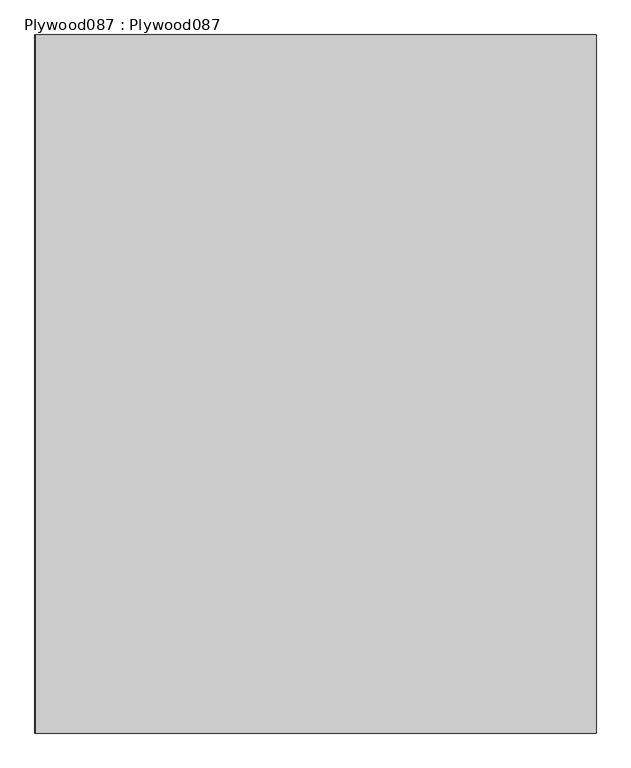
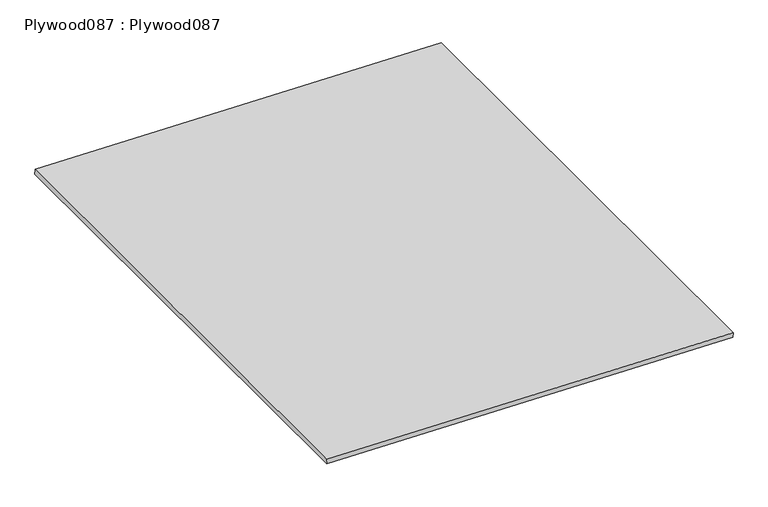
"""IFC4 building model written with IfcOpenShell, lengths in millimetres: proxy geometry, Plywood087 : Plywood087."""

import ifcopenshell
import ifcopenshell.guid

model = None  # the IFC model being written
_history = None  # IfcOwnerHistory: only IFC2X3 demands one
_inside = {}  # id of a spatial element -> (the spatial element, [elements in it])
_under = {}  # id of a project, library or spatial element -> (it, [spatial elements below it])
_declared = {}  # id of a project -> (the project, [libraries it declares])
_typed = {}  # id of a type object -> (the type object, [elements of that type])
_made_of = {}  # id of a material, layer set ... -> (it, [elements and type objects made of it])


def new_model(schema):
    """Start an empty IFC model of exactly this schema.

    Asked for "IFC4X3", IfcOpenShell would pick the latest addendum, in which some entities
    have other attributes; the version numbers below select the first issue.
    IFC2X3 requires an IfcOwnerHistory on every rooted entity: one is made here for all.
    """
    global model, _history
    if schema == "IFC4X3":
        model = ifcopenshell.file(schema_version=(4, 3, 0, 0))
    else:
        model = ifcopenshell.file(schema=schema)
    _inside.clear()
    _under.clear()
    _declared.clear()
    _typed.clear()
    _made_of.clear()
    _history = None
    if model.schema == "IFC2X3":
        org = make("IfcOrganization", Name="unknown")
        user = make(
            "IfcPersonAndOrganization",
            ThePerson=make("IfcPerson", FamilyName="unknown"),
            TheOrganization=org,
        )
        app = make(
            "IfcApplication",
            ApplicationDeveloper=org,
            Version="unknown",
            ApplicationFullName="unknown",
            ApplicationIdentifier="unknown",
        )
        _history = make(
            "IfcOwnerHistory",
            OwningUser=user,
            OwningApplication=app,
            ChangeAction="ADDED",
            CreationDate=0,
        )
    return model


def make(cls, **values):
    """One entity of the class cls with the attributes given. An attribute that is None is left unset."""
    return model.create_entity(
        cls, **{name: value for name, value in values.items() if value is not None}
    )


def rooted(cls, **values):
    """An entity with a GlobalId (a new one), such as an element, a storey or a relation."""
    return make(cls, GlobalId=ifcopenshell.guid.new(), OwnerHistory=_history, **values)


def si_unit(unit_type, name, prefix=None):
    """IfcSIUnit, for example si_unit("LENGTHUNIT", "METRE", prefix="MILLI")."""
    return make("IfcSIUnit", UnitType=unit_type, Prefix=prefix, Name=name)


def assignment(units):
    """IfcUnitAssignment: the units of a project."""
    return None if units is None else make("IfcUnitAssignment", Units=units)


def point(xyz):
    """IfcCartesianPoint."""
    return None if xyz is None else make("IfcCartesianPoint", Coordinates=xyz)


def direction(xyz):
    """IfcDirection."""
    return None if xyz is None else make("IfcDirection", DirectionRatios=xyz)


def frame(location, z_axis=None, x_axis=None):
    """IfcAxis2Placement3D, a coordinate frame: its origin and axes. An axis left out is left unset."""
    return make(
        "IfcAxis2Placement3D",
        Location=point(location),
        Axis=direction(z_axis),
        RefDirection=direction(x_axis),
    )


def origin():
    """The frame at (0, 0, 0) with its axes left unset."""
    return frame((0.0, 0.0, 0.0))


def place(relative_to, where):
    """IfcLocalPlacement: puts the frame where relative to a parent placement (None: the world)."""
    return make(
        "IfcLocalPlacement", PlacementRelTo=relative_to, RelativePlacement=where
    )


def context(
    kind, dimensions, precision=None, world=None, true_north=None, identifier=None
):
    """IfcGeometricRepresentationContext, for example the 3D "Model" context."""
    return make(
        "IfcGeometricRepresentationContext",
        ContextIdentifier=identifier,
        ContextType=kind,
        CoordinateSpaceDimension=dimensions,
        Precision=precision,
        WorldCoordinateSystem=world,
        TrueNorth=true_north,
    )


def project(units=None, contexts=None):
    """IfcProject with its units and contexts."""
    return rooted(
        "IfcProject",
        Name="project",
        RepresentationContexts=contexts,
        UnitsInContext=assignment(units),
    )


def spatial(cls, under=None, at=None, **own):
    """A site, building, storey or space (cls), placed at a placement, below another one or the project."""
    s = rooted(cls, ObjectPlacement=at, **own)
    if under is not None:
        _under.setdefault(under.id(), (under, []))[1].append(s)
    return s


def polyline(points):
    """IfcPolyline through the points."""
    return make("IfcPolyline", Points=[point(p) for p in points])


def outline(outer, holes=None, kind="AREA"):
    """IfcArbitraryClosedProfileDef: a profile drawn as a closed curve; with holes, ...WithVoids."""
    if holes is None:
        return make("IfcArbitraryClosedProfileDef", ProfileType=kind, OuterCurve=outer)
    return make(
        "IfcArbitraryProfileDefWithVoids",
        ProfileType=kind,
        OuterCurve=outer,
        InnerCurves=holes,
    )


def extrude(swept, where, along, depth):
    """IfcExtrudedAreaSolid: the profile swept, set in the frame where, extruded along a direction by depth."""
    return make(
        "IfcExtrudedAreaSolid",
        SweptArea=swept,
        Position=where,
        ExtrudedDirection=direction(along),
        Depth=depth,
    )


def shape(context_of_items, identifier, shape_type, items):
    """IfcShapeRepresentation: the items that make up one representation, for example the "Body"."""
    return make(
        "IfcShapeRepresentation",
        ContextOfItems=context_of_items,
        RepresentationIdentifier=identifier,
        RepresentationType=shape_type,
        Items=items,
    )


def source(mapping_origin, context_of_items, identifier, shape_type, items):
    """IfcRepresentationMap: a shape defined once, which mapped items show again and again."""
    return make(
        "IfcRepresentationMap",
        MappingOrigin=mapping_origin,
        MappedRepresentation=shape(context_of_items, identifier, shape_type, items),
    )


def transform(
    local_origin,
    x_axis=None,
    y_axis=None,
    z_axis=None,
    scale=None,
    scale2=None,
    scale3=None,
    uniform=True,
):
    """IfcCartesianTransformationOperator3D, or its non-uniform kind. x_axis, y_axis, z_axis: its Axis1, 2, 3."""
    if uniform:
        return make(
            "IfcCartesianTransformationOperator3D",
            Axis1=direction(x_axis),
            Axis2=direction(y_axis),
            LocalOrigin=point(local_origin),
            Scale=scale,
            Axis3=direction(z_axis),
        )
    return make(
        "IfcCartesianTransformationOperator3DnonUniform",
        Axis1=direction(x_axis),
        Axis2=direction(y_axis),
        LocalOrigin=point(local_origin),
        Scale=scale,
        Axis3=direction(z_axis),
        Scale2=scale2,
        Scale3=scale3,
    )


def mapped(mapping_source, mapping_target):
    """IfcMappedItem: shows the shape of a source again, moved by a transform."""
    return make(
        "IfcMappedItem", MappingSource=mapping_source, MappingTarget=mapping_target
    )


def made_of(thing, what):
    """Note that an element or type object is made of a material, layer set ...; save() writes the relation."""
    if what is not None:
        _made_of.setdefault(what.id(), (what, []))[1].append(thing)
    return thing


def element(
    cls,
    number,
    at=None,
    inside=None,
    cuts=None,
    type_object=None,
    material=None,
    context=None,
    identifier="Body",
    shape_type=None,
    held_by="IfcProductDefinitionShape",
    body=None,
    shapes=None,
    **own,
):
    """One element of the class cls, such as IfcWall. Its Tag is "e" and its number.

    at: its placement. inside: the storey or other place that contains it. cuts: it is an
    opening in that element (IfcRelVoidsElement). A single representation is given by context,
    identifier, shape_type and body (its items); several are given by shapes. held_by: the class
    of the entity that holds the representations. save() writes the other relations.
    """
    e = rooted(cls, Tag="e%d" % number, ObjectPlacement=at, **own)
    if body is not None:
        shapes = [shape(context, identifier, shape_type, body)]
    if shapes is not None:
        e.Representation = make(held_by, Representations=shapes)
    if inside is not None:
        _inside.setdefault(inside.id(), (inside, []))[1].append(e)
    if cuts is not None:
        rooted(
            "IfcRelVoidsElement", RelatingBuildingElement=cuts, RelatedOpeningElement=e
        )
    if type_object is not None:
        _typed.setdefault(type_object.id(), (type_object, []))[1].append(e)
    return made_of(e, material)


def aggregate(whole, parts):
    """IfcRelAggregates: a whole, such as a stair, and the parts it consists of."""
    return rooted("IfcRelAggregates", RelatingObject=whole, RelatedObjects=parts)


def save(model, path):
    """Write the relations noted so far, then the file.

    IfcRelAggregates (storeys below a building ...), IfcRelContainedInSpatialStructure (elements
    in a storey), IfcRelDefinesByType, IfcRelAssociatesMaterial and IfcRelDeclares: one each for
    every whole, place, type object, material and project.
    """
    for whole, parts in _under.values():
        aggregate(whole, parts)
    for where, things in _inside.values():
        rooted(
            "IfcRelContainedInSpatialStructure",
            RelatedElements=things,
            RelatingStructure=where,
        )
    for kind, things in _typed.values():
        rooted("IfcRelDefinesByType", RelatedObjects=things, RelatingType=kind)
    for what, things in _made_of.values():
        rooted("IfcRelAssociatesMaterial", RelatedObjects=things, RelatingMaterial=what)
    for by, libraries in _declared.values():
        rooted("IfcRelDeclares", RelatingContext=by, RelatedDefinitions=libraries)
    model.write(path)


def plywood087_plywood087_8c4fd348(model_context):
    return source(origin(), model_context, "Body", "SweptSolid", [
        extrude(outline(polyline([(0.0, -1608.7319337), (0.0, 0.0), (2000.0, 0.0), (2000.0, -1608.7319337), (0.0, -1608.7319337)])), frame((-7110.4206035, 7982.1531721, 40101.4890763), z_axis=(0.020896606403401394, 0.0, 0.9997816420803202), x_axis=(0.0, 1.0, 0.0)), (0.0, 0.0, 1.0), 19.05),
    ])


if __name__ == "__main__":
    model = new_model("IFC4")
    model_context = context("Model", 3, world=origin())
    ifc_project = project(units=[si_unit("LENGTHUNIT", "METRE", prefix="MILLI")], contexts=[model_context])
    site = spatial("IfcSite", under=ifc_project)
    building = spatial("IfcBuilding", under=site)
    placement = place(None, origin())
    plywood087_plywood087_shape = plywood087_plywood087_8c4fd348(model_context)
    element("IfcBuildingElementProxy", 1, Name="Plywood087 : Plywood087", ObjectType="Plywood087 : Plywood087", at=placement, inside=building, context=model_context, shape_type="MappedRepresentation", body=[
        mapped(plywood087_plywood087_shape, transform((0.0, 0.0, 0.0), x_axis=(1.0, 0.0, 0.0), y_axis=(0.0, 1.0, 0.0), z_axis=(0.0, 0.0, 1.0))),
    ])
    save(model, "model.ifc")

# Revit data of these elements
# Type "Plywood087 : Plywood087"
#   NameOverride = "Plywood087"
# Element 1 (IfcBuildingElementProxy, "Plywood087 : Plywood087")
#   Materials on its faces: "CDX PLYWOOD -  SEE STRUCTURAL DWGS"
# Materials
#   "CDX PLYWOOD -  SEE STRUCTURAL DWGS": class "Unassigned", colour RGB 177 130 114, transparency 0, Cost = 0
